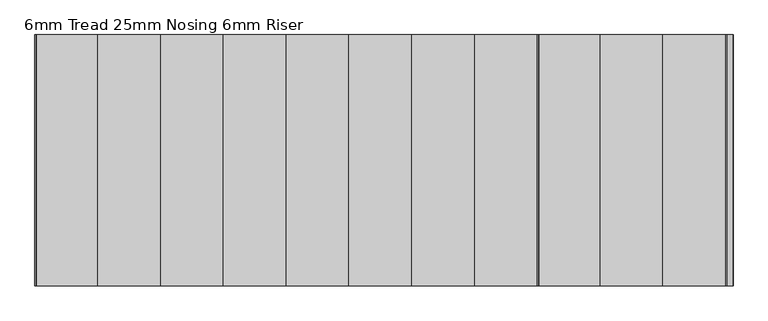
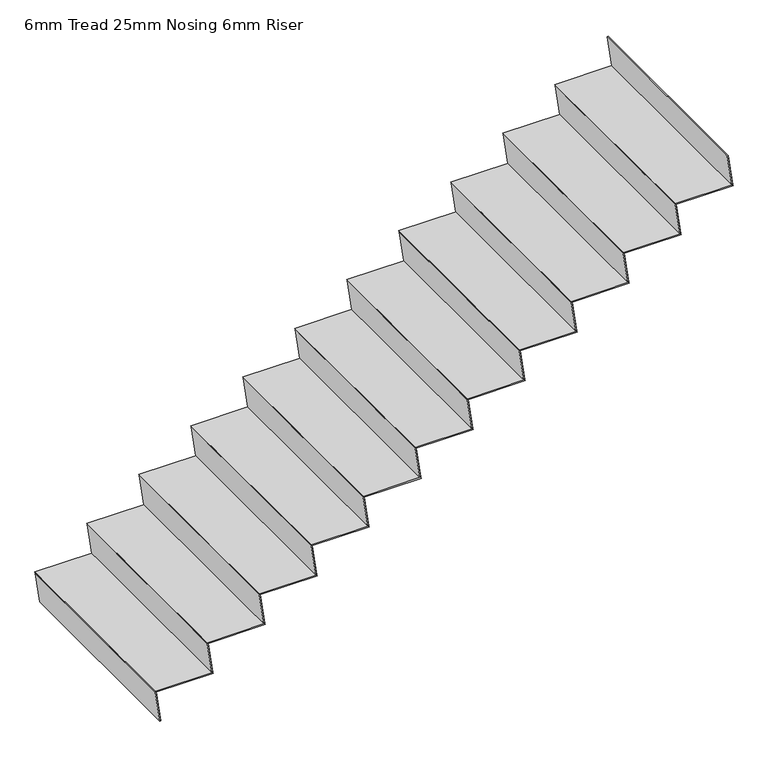
"""IFC4 building model written with IfcOpenShell, lengths in millimetres: stair flight geometry, 6mm Tread 25mm Nosing 6mm Riser."""

from ifc_helpers import new_model, si_unit, frame, origin, place, context, project, spatial, polyline, outline, extrude, source, transform, mapped, element, save


def stair_flight_6mm_tread_25mm_nosing_6mm_riser_8ecd2cec(model_context):
    return source(origin(), model_context, "Body", "SweptSolid", [
        extrude(outline(polyline([(12235.2941176, 13631.0599092), (12235.2941176, 13325.0), (12229.2941176, 13325.85), (12229.2941176, 13631.9099092), (12235.2941176, 13631.0599092)])), frame((0.0, 10370.4345331, 0.0), z_axis=(0.0, 1.0, 0.0), x_axis=(0.0, 0.0, 1.0)), (0.0, 0.0, 1.0), 1100.0),
        extrude(outline(polyline([(12229.2941176, 13325.85), (12058.8235294, 13350.0), (12058.8235294, 13356.0599092), (12229.2941176, 13331.9099092), (12229.2941176, 13325.85)])), frame((0.0, 10370.4345331, 0.0), z_axis=(0.0, 1.0, 0.0), x_axis=(0.0, 0.0, 1.0)), (0.0, 0.0, 1.0), 1100.0),
        extrude(outline(polyline([(12405.7647059, 13600.85), (12235.2941176, 13625.0), (12235.2941176, 13631.0599092), (12405.7647059, 13606.9099092), (12405.7647059, 13600.85)])), frame((0.0, 10370.4345331, 0.0), z_axis=(0.0, 1.0, 0.0), x_axis=(0.0, 0.0, 1.0)), (0.0, 0.0, 1.0), 1100.0),
        extrude(outline(polyline([(12411.7647059, 13906.0599092), (12411.7647059, 13600.0), (12405.7647059, 13600.85), (12405.7647059, 13906.9099092), (12411.7647059, 13906.0599092)])), frame((0.0, 10370.4345331, 0.0), z_axis=(0.0, 1.0, 0.0), x_axis=(0.0, 0.0, 1.0)), (0.0, 0.0, 1.0), 1100.0),
        extrude(outline(polyline([(12582.2352941, 13875.85), (12411.7647059, 13900.0), (12411.7647059, 13906.0599092), (12582.2352941, 13881.9099092), (12582.2352941, 13875.85)])), frame((0.0, 10370.4345331, 0.0), z_axis=(0.0, 1.0, 0.0), x_axis=(0.0, 0.0, 1.0)), (0.0, 0.0, 1.0), 1100.0),
        extrude(outline(polyline([(12588.2352941, 14181.0599092), (12588.2352941, 13875.0), (12582.2352941, 13875.85), (12582.2352941, 14181.9099092), (12588.2352941, 14181.0599092)])), frame((0.0, 10370.4345331, 0.0), z_axis=(0.0, 1.0, 0.0), x_axis=(0.0, 0.0, 1.0)), (0.0, 0.0, 1.0), 1100.0),
        extrude(outline(polyline([(12758.7058824, 14150.85), (12588.2352941, 14175.0), (12588.2352941, 14181.0599092), (12758.7058824, 14156.9099092), (12758.7058824, 14150.85)])), frame((0.0, 10370.4345331, 0.0), z_axis=(0.0, 1.0, 0.0), x_axis=(0.0, 0.0, 1.0)), (0.0, 0.0, 1.0), 1100.0),
        extrude(outline(polyline([(12764.7058824, 14456.0599092), (12764.7058824, 14150.0), (12758.7058824, 14150.85), (12758.7058824, 14456.9099092), (12764.7058824, 14456.0599092)])), frame((0.0, 10370.4345331, 0.0), z_axis=(0.0, 1.0, 0.0), x_axis=(0.0, 0.0, 1.0)), (0.0, 0.0, 1.0), 1100.0),
        extrude(outline(polyline([(12935.1764706, 14425.85), (12764.7058824, 14450.0), (12764.7058824, 14456.0599092), (12935.1764706, 14431.9099092), (12935.1764706, 14425.85)])), frame((0.0, 10370.4345331, 0.0), z_axis=(0.0, 1.0, 0.0), x_axis=(0.0, 0.0, 1.0)), (0.0, 0.0, 1.0), 1100.0),
        extrude(outline(polyline([(12941.1764706, 14731.0599092), (12941.1764706, 14425.0), (12935.1764706, 14425.85), (12935.1764706, 14731.9099092), (12941.1764706, 14731.0599092)])), frame((0.0, 10370.4345331, 0.0), z_axis=(0.0, 1.0, 0.0), x_axis=(0.0, 0.0, 1.0)), (0.0, 0.0, 1.0), 1100.0),
        extrude(outline(polyline([(13111.6470588, 14700.85), (12941.1764706, 14725.0), (12941.1764706, 14731.0599092), (13111.6470588, 14706.9099092), (13111.6470588, 14700.85)])), frame((0.0, 10370.4345331, 0.0), z_axis=(0.0, 1.0, 0.0), x_axis=(0.0, 0.0, 1.0)), (0.0, 0.0, 1.0), 1100.0),
        extrude(outline(polyline([(13117.6470588, 15006.0599092), (13117.6470588, 14700.0), (13111.6470588, 14700.85), (13111.6470588, 15006.9099092), (13117.6470588, 15006.0599092)])), frame((0.0, 10370.4345331, 0.0), z_axis=(0.0, 1.0, 0.0), x_axis=(0.0, 0.0, 1.0)), (0.0, 0.0, 1.0), 1100.0),
        extrude(outline(polyline([(13288.1176471, 14975.85), (13117.6470588, 15000.0), (13117.6470588, 15006.0599092), (13288.1176471, 14981.9099092), (13288.1176471, 14975.85)])), frame((0.0, 10370.4345331, 0.0), z_axis=(0.0, 1.0, 0.0), x_axis=(0.0, 0.0, 1.0)), (0.0, 0.0, 1.0), 1100.0),
        extrude(outline(polyline([(13294.1176471, 15281.0599092), (13294.1176471, 14975.0), (13288.1176471, 14975.85), (13288.1176471, 15281.9099092), (13294.1176471, 15281.0599092)])), frame((0.0, 10370.4345331, 0.0), z_axis=(0.0, 1.0, 0.0), x_axis=(0.0, 0.0, 1.0)), (0.0, 0.0, 1.0), 1100.0),
        extrude(outline(polyline([(13464.5882353, 15250.85), (13294.1176471, 15275.0), (13294.1176471, 15281.0599092), (13464.5882353, 15256.9099092), (13464.5882353, 15250.85)])), frame((0.0, 10370.4345331, 0.0), z_axis=(0.0, 1.0, 0.0), x_axis=(0.0, 0.0, 1.0)), (0.0, 0.0, 1.0), 1100.0),
        extrude(outline(polyline([(13470.5882353, 15556.0599092), (13470.5882353, 15250.0), (13464.5882353, 15250.85), (13464.5882353, 15556.9099092), (13470.5882353, 15556.0599092)])), frame((0.0, 10370.4345331, 0.0), z_axis=(0.0, 1.0, 0.0), x_axis=(0.0, 0.0, 1.0)), (0.0, 0.0, 1.0), 1100.0),
        extrude(outline(polyline([(13641.0588235, 15525.85), (13470.5882353, 15550.0), (13470.5882353, 15556.0599092), (13641.0588235, 15531.9099092), (13641.0588235, 15525.85)])), frame((0.0, 10370.4345331, 0.0), z_axis=(0.0, 1.0, 0.0), x_axis=(0.0, 0.0, 1.0)), (0.0, 0.0, 1.0), 1100.0),
        extrude(outline(polyline([(13647.0588235, 15831.0599092), (13647.0588235, 15525.0), (13641.0588235, 15525.85), (13641.0588235, 15831.9099092), (13647.0588235, 15831.0599092)])), frame((0.0, 10370.4345331, 0.0), z_axis=(0.0, 1.0, 0.0), x_axis=(0.0, 0.0, 1.0)), (0.0, 0.0, 1.0), 1100.0),
        extrude(outline(polyline([(13817.5294118, 15800.85), (13647.0588235, 15825.0), (13647.0588235, 15831.0599092), (13817.5294118, 15806.9099092), (13817.5294118, 15800.85)])), frame((0.0, 10370.4345331, 0.0), z_axis=(0.0, 1.0, 0.0), x_axis=(0.0, 0.0, 1.0)), (0.0, 0.0, 1.0), 1100.0),
        extrude(outline(polyline([(13823.5294118, 16106.0599092), (13823.5294118, 15800.0), (13817.5294118, 15800.85), (13817.5294118, 16106.9099092), (13823.5294118, 16106.0599092)])), frame((0.0, 10370.4345331, 0.0), z_axis=(0.0, 1.0, 0.0), x_axis=(0.0, 0.0, 1.0)), (0.0, 0.0, 1.0), 1100.0),
        extrude(outline(polyline([(13994.0, 16075.85), (13823.5294118, 16100.0), (13823.5294118, 16106.0599092), (13994.0, 16081.9099092), (13994.0, 16075.85)])), frame((0.0, 10370.4345331, 0.0), z_axis=(0.0, 1.0, 0.0), x_axis=(0.0, 0.0, 1.0)), (0.0, 0.0, 1.0), 1100.0),
        extrude(outline(polyline([(14170.4705882, 16350.85), (14000.0, 16375.0), (14000.0, 16381.0599092), (14170.4705882, 16356.9099092), (14170.4705882, 16350.85)])), frame((0.0, 10370.4345331, 0.0), z_axis=(0.0, 1.0, 0.0), x_axis=(0.0, 0.0, 1.0)), (0.0, 0.0, 1.0), 1100.0),
        extrude(outline(polyline([(14000.0, 16381.0599092), (14000.0, 16075.0), (13994.0, 16075.85), (13994.0, 16381.9099092), (14000.0, 16381.0599092)])), frame((0.0, 10370.4345331, 0.0), z_axis=(0.0, 1.0, 0.0), x_axis=(0.0, 0.0, 1.0)), (0.0, 0.0, 1.0), 1100.0),
    ])


if __name__ == "__main__":
    model = new_model("IFC4")
    model_context = context("Model", 3, world=origin())
    ifc_project = project(units=[si_unit("LENGTHUNIT", "METRE", prefix="MILLI")], contexts=[model_context])
    site = spatial("IfcSite", under=ifc_project)
    building = spatial("IfcBuilding", under=site)
    placement = place(None, origin())
    stair_flight_6mm_tread_25mm_nosing_6mm_riser_shape = stair_flight_6mm_tread_25mm_nosing_6mm_riser_8ecd2cec(model_context)
    element("IfcStairFlight", 1, ObjectType="6mm Tread 25mm Nosing 6mm Riser", at=placement, inside=building, context=model_context, shape_type="MappedRepresentation", body=[
        mapped(stair_flight_6mm_tread_25mm_nosing_6mm_riser_shape, transform((0.0, 0.0, 0.0), x_axis=(1.0, 0.0, 0.0), y_axis=(0.0, 1.0, 0.0), z_axis=(0.0, 0.0, 1.0))),
    ])
    save(model, "model.ifc")

# Revit data of these elements
# Element 1 (IfcStairFlight, "6mm Tread 25mm Nosing 6mm Riser")
#   Materials on its faces: "Steel, Paint Finish, Dark Gray"
# Materials
#   "Steel, Paint Finish, Dark Gray": class "Metal", colour RGB 89 89 89, transparency 0, Description = "Steel, paint finish, dark gray, glossy", Cost = 0
